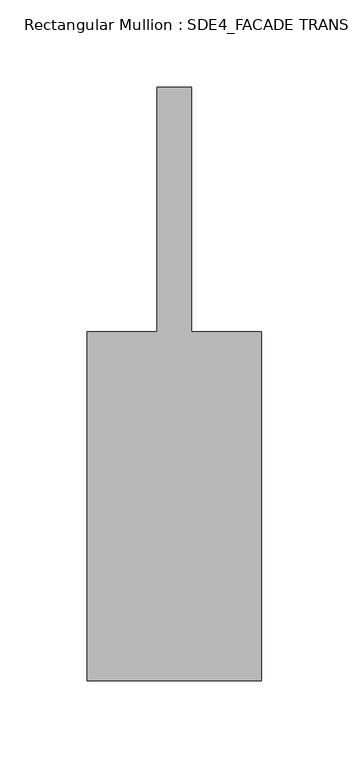
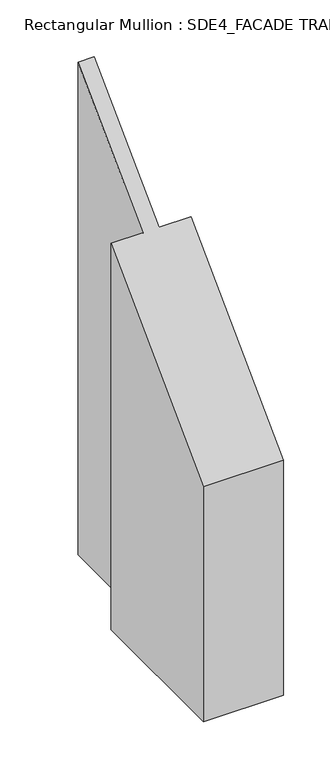
"""IFC4 building model written with IfcOpenShell, lengths in millimetres: member geometry, Rectangular Mullion : SDE4_FACADE TRANSOM TYPE 1."""

from ifc_helpers import new_model, si_unit, origin, place, context, project, spatial, faceted_brep, source, transform, mapped, element, save


def rectangular_mullion_sde4_facade_transom_type_1_936a2651(model_context):
    return source(origin(), model_context, "Body", "Brep", [
        faceted_brep([(50.0, -132.5, -442.1403747), (-50.0, -132.5, -442.1403747), (-50.0, 67.5, -442.1403747), (-10.0, 67.5, -442.1403747), (-10.0, 207.5, -442.1403747), (10.0, 207.5, -442.1403747), (10.0, 67.5, -442.1403747), (50.0, 67.5, -442.1403747), (50.0, 67.5, 67.5), (50.0, -132.5, -132.5), (10.0, 67.5, 67.5), (10.0, 207.5, 207.5), (-10.0, 207.5, 207.5), (-10.0, 67.5, 67.5), (-50.0, 67.5, 67.5), (-50.0, -132.5, -132.5)], [[[0, 1, 2, 3, 4, 5, 6, 7]], [[8, 9, 0, 7]], [[10, 8, 7, 6]], [[11, 10, 6, 5]], [[12, 11, 5, 4]], [[13, 12, 4, 3]], [[14, 13, 3, 2]], [[15, 14, 2, 1]], [[9, 15, 1, 0]], [[9, 8, 10, 11, 12, 13, 14, 15]]]),
    ])


if __name__ == "__main__":
    model = new_model("IFC4")
    model_context = context("Model", 3, world=origin())
    ifc_project = project(units=[si_unit("LENGTHUNIT", "METRE", prefix="MILLI")], contexts=[model_context])
    site = spatial("IfcSite", under=ifc_project)
    building = spatial("IfcBuilding", under=site)
    placement = place(None, origin())
    rectangular_mullion_sde4_facade_transom_type_1_shape = rectangular_mullion_sde4_facade_transom_type_1_936a2651(model_context)
    element("IfcMember", 1, ObjectType="Rectangular Mullion : SDE4_FACADE TRANSOM TYPE 1", at=placement, inside=building, context=model_context, shape_type="MappedRepresentation", body=[
        mapped(rectangular_mullion_sde4_facade_transom_type_1_shape, transform((0.0, 0.0, 0.0), x_axis=(1.0, 0.0, 0.0), y_axis=(0.0, 1.0, 0.0), z_axis=(0.0, 0.0, 1.0))),
    ])
    save(model, "model.ifc")

# Revit data of these elements
# Type "Rectangular Mullion : SDE4_FACADE TRANSOM TYPE 1"
#   built-in parameter 1007322 = 1.11549 (stored number, unit not read)
#   built-in parameter 1007321 = 0.164042 (stored number, unit not read)
#   built-in parameter 1007320 = 0.164042 (stored number, unit not read)
